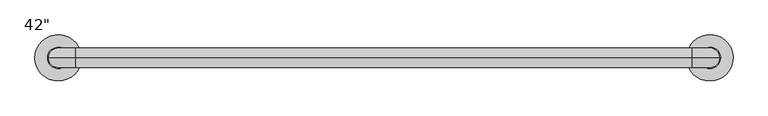
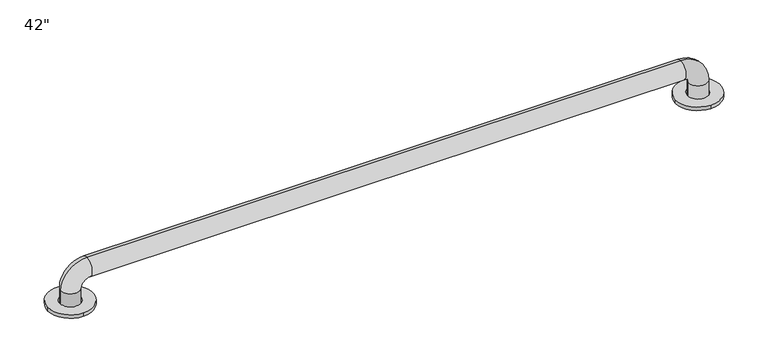
"""IFC4 building model written with IfcOpenShell, lengths in millimetres: proxy geometry."""

import ifcopenshell
import ifcopenshell.guid

model = None  # the IFC model being written
_history = None  # IfcOwnerHistory: only IFC2X3 demands one
_inside = {}  # id of a spatial element -> (the spatial element, [elements in it])
_under = {}  # id of a project, library or spatial element -> (it, [spatial elements below it])
_declared = {}  # id of a project -> (the project, [libraries it declares])
_typed = {}  # id of a type object -> (the type object, [elements of that type])
_made_of = {}  # id of a material, layer set ... -> (it, [elements and type objects made of it])


def new_model(schema):
    """Start an empty IFC model of exactly this schema.

    Asked for "IFC4X3", IfcOpenShell would pick the latest addendum, in which some entities
    have other attributes; the version numbers below select the first issue.
    IFC2X3 requires an IfcOwnerHistory on every rooted entity: one is made here for all.
    """
    global model, _history
    if schema == "IFC4X3":
        model = ifcopenshell.file(schema_version=(4, 3, 0, 0))
    else:
        model = ifcopenshell.file(schema=schema)
    _inside.clear()
    _under.clear()
    _declared.clear()
    _typed.clear()
    _made_of.clear()
    _history = None
    if model.schema == "IFC2X3":
        org = make("IfcOrganization", Name="unknown")
        user = make(
            "IfcPersonAndOrganization",
            ThePerson=make("IfcPerson", FamilyName="unknown"),
            TheOrganization=org,
        )
        app = make(
            "IfcApplication",
            ApplicationDeveloper=org,
            Version="unknown",
            ApplicationFullName="unknown",
            ApplicationIdentifier="unknown",
        )
        _history = make(
            "IfcOwnerHistory",
            OwningUser=user,
            OwningApplication=app,
            ChangeAction="ADDED",
            CreationDate=0,
        )
    return model


def make(cls, **values):
    """One entity of the class cls with the attributes given. An attribute that is None is left unset."""
    return model.create_entity(
        cls, **{name: value for name, value in values.items() if value is not None}
    )


def rooted(cls, **values):
    """An entity with a GlobalId (a new one), such as an element, a storey or a relation."""
    return make(cls, GlobalId=ifcopenshell.guid.new(), OwnerHistory=_history, **values)


def si_unit(unit_type, name, prefix=None):
    """IfcSIUnit, for example si_unit("LENGTHUNIT", "METRE", prefix="MILLI")."""
    return make("IfcSIUnit", UnitType=unit_type, Prefix=prefix, Name=name)


def assignment(units):
    """IfcUnitAssignment: the units of a project."""
    return None if units is None else make("IfcUnitAssignment", Units=units)


def point(xyz):
    """IfcCartesianPoint."""
    return None if xyz is None else make("IfcCartesianPoint", Coordinates=xyz)


def direction(xyz):
    """IfcDirection."""
    return None if xyz is None else make("IfcDirection", DirectionRatios=xyz)


def frame(location, z_axis=None, x_axis=None):
    """IfcAxis2Placement3D, a coordinate frame: its origin and axes. An axis left out is left unset."""
    return make(
        "IfcAxis2Placement3D",
        Location=point(location),
        Axis=direction(z_axis),
        RefDirection=direction(x_axis),
    )


def frame_2d(location, x_axis=None):
    """IfcAxis2Placement2D, a coordinate frame in the plane: its origin and x axis."""
    return make(
        "IfcAxis2Placement2D", Location=point(location), RefDirection=direction(x_axis)
    )


def origin():
    """The frame at (0, 0, 0) with its axes left unset."""
    return frame((0.0, 0.0, 0.0))


def origin_with_axes():
    """The frame at (0, 0, 0) with the z axis (0, 0, 1) and the x axis (1, 0, 0) written out."""
    return frame((0.0, 0.0, 0.0), z_axis=(0.0, 0.0, 1.0), x_axis=(1.0, 0.0, 0.0))


def origin_2d():
    """The frame at (0, 0) in the plane with its x axis left unset."""
    return frame_2d((0.0, 0.0))


def place(relative_to, where):
    """IfcLocalPlacement: puts the frame where relative to a parent placement (None: the world)."""
    return make(
        "IfcLocalPlacement", PlacementRelTo=relative_to, RelativePlacement=where
    )


def context(
    kind, dimensions, precision=None, world=None, true_north=None, identifier=None
):
    """IfcGeometricRepresentationContext, for example the 3D "Model" context."""
    return make(
        "IfcGeometricRepresentationContext",
        ContextIdentifier=identifier,
        ContextType=kind,
        CoordinateSpaceDimension=dimensions,
        Precision=precision,
        WorldCoordinateSystem=world,
        TrueNorth=true_north,
    )


def project(units=None, contexts=None):
    """IfcProject with its units and contexts."""
    return rooted(
        "IfcProject",
        Name="project",
        RepresentationContexts=contexts,
        UnitsInContext=assignment(units),
    )


def spatial(cls, under=None, at=None, **own):
    """A site, building, storey or space (cls), placed at a placement, below another one or the project."""
    s = rooted(cls, ObjectPlacement=at, **own)
    if under is not None:
        _under.setdefault(under.id(), (under, []))[1].append(s)
    return s


def circle_curve(where, radius):
    """IfcCircle in the frame where."""
    return make("IfcCircle", Position=where, Radius=radius)


def ellipse_curve(where, semi_axis1, semi_axis2):
    """IfcEllipse in the frame where."""
    return make(
        "IfcEllipse", Position=where, SemiAxis1=semi_axis1, SemiAxis2=semi_axis2
    )


def trimmed(basis, trim1, trim2, sense, master):
    """IfcTrimmedCurve: the piece of a basis curve between two trims."""
    return make(
        "IfcTrimmedCurve",
        BasisCurve=basis,
        Trim1=trim1,
        Trim2=trim2,
        SenseAgreement=sense,
        MasterRepresentation=master,
    )


def segment(curve, same_sense, transition):
    """IfcCompositeCurveSegment."""
    return make(
        "IfcCompositeCurveSegment",
        Transition=transition,
        SameSense=same_sense,
        ParentCurve=curve,
    )


def composite_curve(segments, self_intersect=None):
    """IfcCompositeCurve: segments joined end to end."""
    return make("IfcCompositeCurve", Segments=segments, SelfIntersect=self_intersect)


def outline(outer, holes=None, kind="AREA"):
    """IfcArbitraryClosedProfileDef: a profile drawn as a closed curve; with holes, ...WithVoids."""
    if holes is None:
        return make("IfcArbitraryClosedProfileDef", ProfileType=kind, OuterCurve=outer)
    return make(
        "IfcArbitraryProfileDefWithVoids",
        ProfileType=kind,
        OuterCurve=outer,
        InnerCurves=holes,
    )


def extrude(swept, where, along, depth):
    """IfcExtrudedAreaSolid: the profile swept, set in the frame where, extruded along a direction by depth."""
    return make(
        "IfcExtrudedAreaSolid",
        SweptArea=swept,
        Position=where,
        ExtrudedDirection=direction(along),
        Depth=depth,
    )


def shape(context_of_items, identifier, shape_type, items):
    """IfcShapeRepresentation: the items that make up one representation, for example the "Body"."""
    return make(
        "IfcShapeRepresentation",
        ContextOfItems=context_of_items,
        RepresentationIdentifier=identifier,
        RepresentationType=shape_type,
        Items=items,
    )


def source(mapping_origin, context_of_items, identifier, shape_type, items):
    """IfcRepresentationMap: a shape defined once, which mapped items show again and again."""
    return make(
        "IfcRepresentationMap",
        MappingOrigin=mapping_origin,
        MappedRepresentation=shape(context_of_items, identifier, shape_type, items),
    )


def transform(
    local_origin,
    x_axis=None,
    y_axis=None,
    z_axis=None,
    scale=None,
    scale2=None,
    scale3=None,
    uniform=True,
):
    """IfcCartesianTransformationOperator3D, or its non-uniform kind. x_axis, y_axis, z_axis: its Axis1, 2, 3."""
    if uniform:
        return make(
            "IfcCartesianTransformationOperator3D",
            Axis1=direction(x_axis),
            Axis2=direction(y_axis),
            LocalOrigin=point(local_origin),
            Scale=scale,
            Axis3=direction(z_axis),
        )
    return make(
        "IfcCartesianTransformationOperator3DnonUniform",
        Axis1=direction(x_axis),
        Axis2=direction(y_axis),
        LocalOrigin=point(local_origin),
        Scale=scale,
        Axis3=direction(z_axis),
        Scale2=scale2,
        Scale3=scale3,
    )


def mapped(mapping_source, mapping_target):
    """IfcMappedItem: shows the shape of a source again, moved by a transform."""
    return make(
        "IfcMappedItem", MappingSource=mapping_source, MappingTarget=mapping_target
    )


def made_of(thing, what):
    """Note that an element or type object is made of a material, layer set ...; save() writes the relation."""
    if what is not None:
        _made_of.setdefault(what.id(), (what, []))[1].append(thing)
    return thing


def element(
    cls,
    number,
    at=None,
    inside=None,
    cuts=None,
    type_object=None,
    material=None,
    context=None,
    identifier="Body",
    shape_type=None,
    held_by="IfcProductDefinitionShape",
    body=None,
    shapes=None,
    **own,
):
    """One element of the class cls, such as IfcWall. Its Tag is "e" and its number.

    at: its placement. inside: the storey or other place that contains it. cuts: it is an
    opening in that element (IfcRelVoidsElement). A single representation is given by context,
    identifier, shape_type and body (its items); several are given by shapes. held_by: the class
    of the entity that holds the representations. save() writes the other relations.
    """
    e = rooted(cls, Tag="e%d" % number, ObjectPlacement=at, **own)
    if body is not None:
        shapes = [shape(context, identifier, shape_type, body)]
    if shapes is not None:
        e.Representation = make(held_by, Representations=shapes)
    if inside is not None:
        _inside.setdefault(inside.id(), (inside, []))[1].append(e)
    if cuts is not None:
        rooted(
            "IfcRelVoidsElement", RelatingBuildingElement=cuts, RelatedOpeningElement=e
        )
    if type_object is not None:
        _typed.setdefault(type_object.id(), (type_object, []))[1].append(e)
    return made_of(e, material)


def aggregate(whole, parts):
    """IfcRelAggregates: a whole, such as a stair, and the parts it consists of."""
    return rooted("IfcRelAggregates", RelatingObject=whole, RelatedObjects=parts)


def save(model, path):
    """Write the relations noted so far, then the file.

    IfcRelAggregates (storeys below a building ...), IfcRelContainedInSpatialStructure (elements
    in a storey), IfcRelDefinesByType, IfcRelAssociatesMaterial and IfcRelDeclares: one each for
    every whole, place, type object, material and project.
    """
    for whole, parts in _under.values():
        aggregate(whole, parts)
    for where, things in _inside.values():
        rooted(
            "IfcRelContainedInSpatialStructure",
            RelatedElements=things,
            RelatingStructure=where,
        )
    for kind, things in _typed.values():
        rooted("IfcRelDefinesByType", RelatedObjects=things, RelatingType=kind)
    for what, things in _made_of.values():
        rooted("IfcRelAssociatesMaterial", RelatedObjects=things, RelatingMaterial=what)
    for by, libraries in _declared.values():
        rooted("IfcRelDeclares", RelatingContext=by, RelatedDefinitions=libraries)
    model.write(path)


def plane_surface(at):
    """IfcPlane: the flat surface through the origin of the frame at, square to its z axis."""
    return make("IfcPlane", Position=at)


def cylinder_surface(at, radius):
    """IfcCylindricalSurface: all points at the distance radius from the z axis of the frame at."""
    return make("IfcCylindricalSurface", Position=at, Radius=radius)


def revolved_surface(curve, axis_point, axis_direction):
    """IfcSurfaceOfRevolution: the curve turned about the line through axis_point along axis_direction."""
    return make(
        "IfcSurfaceOfRevolution",
        SweptCurve=make("IfcArbitraryOpenProfileDef", ProfileType="CURVE", Curve=curve),
        AxisPosition=make("IfcAxis1Placement", Location=point(axis_point), Axis=direction(axis_direction)),
    )


def advanced_brep(points, edges, surfaces, faces):
    """IfcAdvancedBrep: a solid bounded by faces that lie on surfaces and meet in shared edges.

    An edge is (start, end): straight between two places in points (the first is 0);
    or (start, end, curve); or (start, end, curve, False) where it runs against its curve.
    A face is (place in surfaces, loops), or (place, loops, False) where it looks against
    its surface's normal. A loop lists edges by number (the first is 1), with a minus sign
    where the edge is run from its end to its start. The first loop is the outer one.
    """
    corners = [point(p) for p in points]
    vertices = [make("IfcVertexPoint", VertexGeometry=c) for c in corners]
    made = []
    for start, end, *more in edges:
        made.append(
            make(
                "IfcEdgeCurve",
                EdgeStart=vertices[start],
                EdgeEnd=vertices[end],
                EdgeGeometry=more[0] if more else make("IfcPolyline", Points=[corners[start], corners[end]]),
                SameSense=more[1] if len(more) > 1 else True,
            )
        )
    hull = []
    for where, loops, *sense in faces:
        bounds = []
        for j, loop in enumerate(loops):
            ring = [make("IfcOrientedEdge", EdgeElement=made[abs(k) - 1], Orientation=k > 0) for k in loop]
            bounds.append(
                make(
                    "IfcFaceOuterBound" if j == 0 else "IfcFaceBound",
                    Bound=make("IfcEdgeLoop", EdgeList=ring),
                    Orientation=True,
                )
            )
        hull.append(make("IfcAdvancedFace", Bounds=bounds, FaceSurface=surfaces[where], SameSense=sense[0] if sense else True))
    return make("IfcAdvancedBrep", Outer=make("IfcClosedShell", CfsFaces=hull))


def proxy_a4e7295d(model_context):
    return source(origin(), model_context, "Body", "SolidModel", [
        extrude(outline(composite_curve([segment(trimmed(circle_curve(frame_2d((1066.8, 0.0)), 38.1), [point((1028.7, 0.0))], [point((1066.8, -38.1))], False, "CARTESIAN"), True, "CONTINUOUS"), segment(trimmed(circle_curve(frame_2d((1066.8, 0.0)), 38.1), [point((1066.8, -38.1))], [point((1028.7, 0.0))], False, "CARTESIAN"), True, "CONTINUOUS")], self_intersect=False), holes=[composite_curve([segment(trimmed(circle_curve(frame_2d((1066.8, 0.0)), 17.4625), [point((1049.3375, 0.0))], [point((1066.8, -17.4625))], True, "CARTESIAN"), True, "CONTINUOUS"), segment(trimmed(circle_curve(frame_2d((1066.8, 0.0)), 17.4625), [point((1066.8, -17.4625))], [point((1049.3375, 0.0))], True, "CARTESIAN"), True, "CONTINUOUS")], self_intersect=False)]), origin_with_axes(), (0.0, 0.0, 1.0), 6.35),
        extrude(outline(composite_curve([segment(trimmed(circle_curve(origin_2d(), 38.1), [point((-38.1, 0.0))], [point((0.0, -38.1))], False, "CARTESIAN"), True, "CONTINUOUS"), segment(trimmed(circle_curve(origin_2d(), 38.1), [point((0.0, -38.1))], [point((-38.1, 0.0))], False, "CARTESIAN"), True, "CONTINUOUS")], self_intersect=False), holes=[composite_curve([segment(trimmed(circle_curve(origin_2d(), 17.4625), [point((-17.4625, 0.0))], [point((0.0, -17.4625))], True, "CARTESIAN"), True, "CONTINUOUS"), segment(trimmed(circle_curve(origin_2d(), 17.4625), [point((0.0, -17.4625))], [point((-17.4625, 0.0))], True, "CARTESIAN"), True, "CONTINUOUS")], self_intersect=False)]), origin_with_axes(), (0.0, 0.0, 1.0), 6.35),
        advanced_brep(
        [(1082.675, 0.0, 0.0), (1050.925, 0.0, 0.0), (1082.675, 0.0, 28.575), (1050.925, 0.0, 28.575), (1038.225, 0.0, 41.275), (1038.225, 0.0, 73.025), (28.575, 0.0, 73.025), (28.575, 0.0, 41.275), (15.875, 0.0, 28.575), (-15.875, 0.0, 28.575), (-15.875, 0.0, 0.0), (15.875, 0.0, 0.0)],
        [
            (0, 1, circle_curve(frame((1066.8, 0.0, 0.0), z_axis=(0.0, 0.0, -1.0), x_axis=(-1.0, 0.0, 0.0)), 15.875)),
            (1, 0, circle_curve(frame((1066.8, 0.0, 0.0), z_axis=(0.0, 0.0, -1.0), x_axis=(-1.0, 0.0, 0.0)), 15.875)),
            (0, 2),
            (2, 3, circle_curve(frame((1066.8, 0.0, 28.575), z_axis=(0.0, 0.0, -1.0), x_axis=(-1.0, 0.0, 0.0)), 15.875)),
            (3, 1),
            (3, 2, circle_curve(frame((1066.8, 0.0, 28.575), z_axis=(0.0, 0.0, -1.0), x_axis=(-1.0, 0.0, 0.0)), 15.875)),
            (4, 3, circle_curve(frame((1038.225, 0.0, 28.575), z_axis=(0.0, 1.0, 0.0), x_axis=(1.0, 0.0, 0.0)), 12.7)),
            (2, 5, circle_curve(frame((1038.225, 0.0, 28.575), z_axis=(0.0, -1.0, 0.0), x_axis=(1.0, 0.0, 0.0)), 44.45)),
            (5, 4, circle_curve(frame((1038.225, 0.0, 57.15), z_axis=(1.0, 0.0, 0.0), x_axis=(0.0, 0.0, -1.0)), 15.875)),
            (4, 5, circle_curve(frame((1038.225, 0.0, 57.15), z_axis=(1.0, 0.0, 0.0), x_axis=(0.0, 0.0, -1.0)), 15.875)),
            (5, 6),
            (6, 7, circle_curve(frame((28.575, 0.0, 57.15), z_axis=(1.0, 0.0, 0.0), x_axis=(0.0, 0.0, -1.0)), 15.875)),
            (7, 4),
            (7, 6, circle_curve(frame((28.575, 0.0, 57.15), z_axis=(1.0, 0.0, 0.0), x_axis=(0.0, 0.0, -1.0)), 15.875)),
            (8, 7, circle_curve(frame((28.575, 0.0, 28.575), z_axis=(0.0, 1.0, 0.0), x_axis=(0.0, 0.0, 1.0)), 12.7)),
            (6, 9, circle_curve(frame((28.575, 0.0, 28.575), z_axis=(0.0, -1.0, 0.0), x_axis=(0.0, 0.0, 1.0)), 44.45)),
            (9, 8, circle_curve(frame((0.0, 0.0, 28.575), z_axis=(0.0, 0.0, 1.0), x_axis=(1.0, 0.0, 0.0)), 15.875)),
            (8, 9, circle_curve(frame((0.0, 0.0, 28.575), z_axis=(0.0, 0.0, 1.0), x_axis=(1.0, 0.0, 0.0)), 15.875)),
            (10, 11, circle_curve(frame((0.0, 0.0, 0.0), z_axis=(0.0, 0.0, -1.0), x_axis=(1.0, 0.0, 0.0)), 15.875)),
            (11, 10, circle_curve(frame((0.0, 0.0, 0.0), z_axis=(0.0, 0.0, -1.0), x_axis=(1.0, 0.0, 0.0)), 15.875)),
            (9, 10),
            (11, 8),
        ],
        [
            plane_surface(frame((1066.8, 0.0, 0.0), z_axis=(0.0, 0.0, -1.0), x_axis=(0.0, -1.0, 0.0))),
            cylinder_surface(frame((1066.8, 0.0, 0.0), z_axis=(0.0, 0.0, -1.0), x_axis=(-1.0, 0.0, 0.0)), 15.875),
            revolved_surface(trimmed(ellipse_curve(frame((1066.8, 0.0, 28.575), z_axis=(0.0, 0.0, -1.0), x_axis=(-1.0, 0.0, 0.0)), 15.875, 15.875), [point((1082.675, 0.0, 28.575))], [point((1050.925, 0.0, 28.575))], True, "CARTESIAN"), (1038.225, 0.0, 28.575), (0.0, -1.0, 0.0)),
            revolved_surface(trimmed(ellipse_curve(frame((1066.8, 0.0, 28.575), z_axis=(0.0, 0.0, -1.0), x_axis=(-1.0, 0.0, 0.0)), 15.875, 15.875), [point((1050.925, 0.0, 28.575))], [point((1082.675, 0.0, 28.575))], True, "CARTESIAN"), (1038.225, 0.0, 28.575), (0.0, -1.0, 0.0)),
            cylinder_surface(frame((1038.225, 0.0, 57.15), z_axis=(1.0, 0.0, 0.0), x_axis=(0.0, 0.0, -1.0)), 15.875),
            revolved_surface(trimmed(ellipse_curve(frame((28.575, 0.0, 57.15), z_axis=(1.0, 0.0, 0.0), x_axis=(0.0, 0.0, -1.0)), 15.875, 15.875), [point((28.575, 0.0, 73.025))], [point((28.575, 0.0, 41.275))], True, "CARTESIAN"), (28.575, 0.0, 28.575), (0.0, -1.0, 0.0)),
            revolved_surface(trimmed(ellipse_curve(frame((28.575, 0.0, 57.15), z_axis=(1.0, 0.0, 0.0), x_axis=(0.0, 0.0, -1.0)), 15.875, 15.875), [point((28.575, 0.0, 41.275))], [point((28.575, 0.0, 73.025))], True, "CARTESIAN"), (28.575, 0.0, 28.575), (0.0, -1.0, 0.0)),
            plane_surface(frame((0.0, 0.0, 0.0), z_axis=(0.0, 0.0, -1.0), x_axis=(0.0, -1.0, 0.0))),
            cylinder_surface(frame((0.0, 0.0, 28.575), z_axis=(0.0, 0.0, 1.0), x_axis=(1.0, 0.0, 0.0)), 15.875),
        ],
        [
            (0, [[1, 2]]),
            (1, [[-1, 3, 4, 5]]),
            (1, [[-2, -5, 6, -3]]),
            (2, [[7, -4, 8, 9]]),
            (3, [[-8, -6, -7, 10]]),
            (4, [[-9, 11, 12, 13]]),
            (4, [[-10, -13, 14, -11]]),
            (5, [[15, -12, 16, 17]]),
            (6, [[-16, -14, -15, 18]]),
            (7, [[19, 20]]),
            (8, [[-17, 21, -20, 22]]),
            (8, [[-18, -22, -19, -21]]),
        ],
    ),
    ])


if __name__ == "__main__":
    model = new_model("IFC4")
    model_context = context("Model", 3, world=origin())
    ifc_project = project(units=[si_unit("LENGTHUNIT", "METRE", prefix="MILLI")], contexts=[model_context])
    site = spatial("IfcSite", under=ifc_project)
    building = spatial("IfcBuilding", under=site)
    placement = place(None, origin())
    proxy_shape = proxy_a4e7295d(model_context)
    element("IfcBuildingElementProxy", 1, Name="Seqm-Grab Bar : 42\"", ObjectType="Seqm-Grab Bar : 42\"", at=placement, inside=building, context=model_context, shape_type="MappedRepresentation", body=[
        mapped(proxy_shape, transform((0.0, 0.0, 0.0), x_axis=(1.0, 0.0, 0.0), y_axis=(0.0, 1.0, 0.0), z_axis=(0.0, 0.0, 1.0))),
    ])
    save(model, "model.ifc")

# Revit data of these elements
# Type "Seqm-Grab Bar : 42\""
#   Spec Number = "10 28 00"
#   Spec Description = "42\" GRAB BAR"
#   Length = 3' - 6"
#   Default Elevation = 4' - 0"
#   Grab Bar Material = GRAB BARS - AT ADA RESTROOMS ONLY
# Element 1 (IfcBuildingElementProxy, "Seqm-Grab Bar : 42\"")
#   Materials on its faces: "GRAB BARS - AT ADA RESTROOMS ONLY"
# Materials
#   "GRAB BARS - AT ADA RESTROOMS ONLY": class "Generic", colour RGB 120 120 120, transparency 0, Cost = 0
